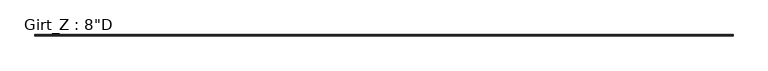
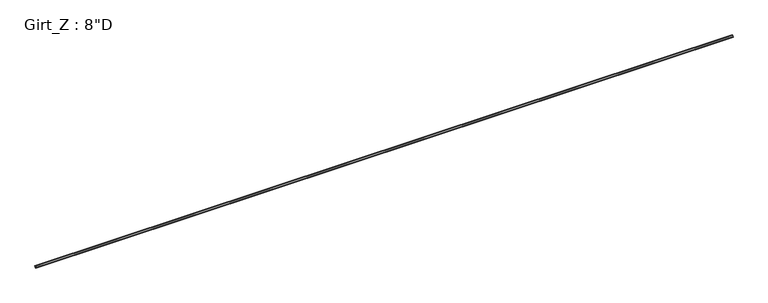
"""IFC4 building model written with IfcOpenShell, lengths in millimetres: beam geometry."""

from ifc_helpers import new_model, si_unit, point, frame, frame_2d, origin, place, context, project, spatial, polyline, circle_curve, trimmed, segment, composite_curve, outline, extrude, source, transform, mapped, element, save


def beam_a5903320(model_context):
    return source(origin(), model_context, "Body", "SweptSolid", [
        extrude(outline(composite_curve([segment(polyline([(63.5, 101.6), (75.745104, 87.0068534), (73.6169367, 85.221109), (62.204539, 98.821875), (3.3005807, 98.821875)]), True, "CONTINUOUS"), segment(trimmed(circle_curve(frame_2d((3.3741066, 96.8381931)), 1.9850441), [point((3.3005807, 98.821875))], [point((1.3890625, 96.8381931))], True, "CARTESIAN"), True, "CONTINUOUS"), segment(polyline([(1.3890625, 96.8381931), (1.3890625, -96.8375)]), True, "CONTINUOUS"), segment(trimmed(circle_curve(frame_2d((-3.3734375, -96.8375)), 4.7625), [point((1.3890625, -96.8375))], [point((-3.3734375, -101.6))], False, "CARTESIAN"), True, "CONTINUOUS"), segment(polyline([(-3.3734375, -101.6), (-63.5, -101.6), (-75.745104, -87.0068534), (-73.6169367, -85.221109), (-62.204539, -98.821875), (-3.2694106, -98.821875)]), True, "CONTINUOUS"), segment(trimmed(circle_curve(frame_2d((-3.3748024, -96.8389339)), 1.9857399), [point((-3.2694106, -98.821875))], [point((-1.3890625, -96.8389339))], True, "CARTESIAN"), True, "CONTINUOUS"), segment(polyline([(-1.3890625, -96.8389339), (-1.3890625, 96.8375)]), True, "CONTINUOUS"), segment(trimmed(circle_curve(frame_2d((3.3734375, 96.8375)), 4.7625), [point((-1.3890625, 96.8375))], [point((3.3734375, 101.6))], False, "CARTESIAN"), True, "CONTINUOUS"), segment(polyline([(3.3734375, 101.6), (63.5, 101.6)]), True, "CONTINUOUS")], self_intersect=False)), frame((-44156.1884766, 0.0, 0.0), z_axis=(1.0, 0.0, 0.0), x_axis=(0.0, 1.0, 0.0)), (0.0, 0.0, 1.0), 88312.3769531),
    ])


if __name__ == "__main__":
    model = new_model("IFC4")
    model_context = context("Model", 3, world=origin())
    ifc_project = project(units=[si_unit("LENGTHUNIT", "METRE", prefix="MILLI")], contexts=[model_context])
    site = spatial("IfcSite", under=ifc_project)
    building = spatial("IfcBuilding", under=site)
    placement = place(None, origin())
    beam_shape = beam_a5903320(model_context)
    element("IfcBeam", 1, ObjectType="Girt_Z : 8\"D", at=placement, inside=building, context=model_context, shape_type="MappedRepresentation", body=[
        mapped(beam_shape, transform((0.0, 0.0, 0.0), x_axis=(1.0, 0.0, 0.0), y_axis=(0.0, 1.0, 0.0), z_axis=(0.0, 0.0, 1.0))),
    ])
    save(model, "model.ifc")

# Revit data of these elements
# Type "Girt_Z : 8\"D"
#   Web_Thickness = 0' - 0 7/64"
#   Length [instance default] = 10' - 0"
#   Leg_1 = 0' - 2 1/2"
#   Height = 0' - 8"
#   Structural Material [instance default] = none
